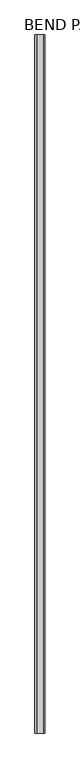
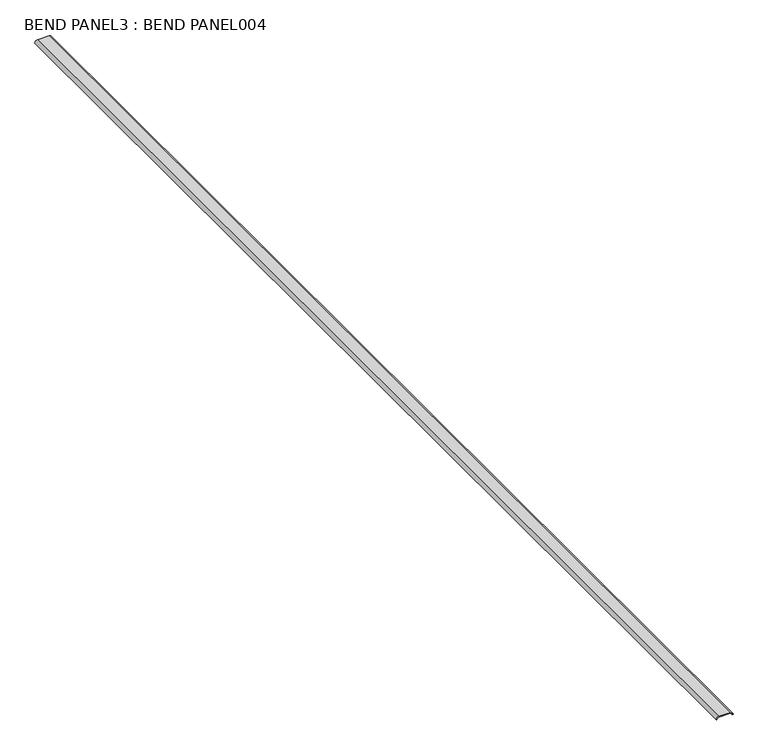
"""IFC4 building model written with IfcOpenShell, lengths in millimetres: proxy geometry, BEND PANEL3 : BEND PANEL004."""

from ifc_helpers import new_model, si_unit, point, frame, frame_2d, origin, place, context, project, spatial, polyline, circle_curve, trimmed, segment, composite_curve, outline, extrude, source, transform, mapped, element, save


def bend_panel3_bend_panel004_15d214a6(model_context):
    return source(origin(), model_context, "Body", "SweptSolid", [
        extrude(outline(composite_curve([segment(polyline([(42576.61192, 5858.4004637), (42576.61192, 5859.5910887)]), True, "CONTINUOUS"), segment(trimmed(circle_curve(frame_2d((42576.6119199, 5862.9993652)), 3.4082764), [point((42576.61192, 5859.5910887))], [point((42580.0201795, 5863.0100787))], True, "CARTESIAN"), True, "CONTINUOUS"), segment(polyline([(42580.0201795, 5863.0100787), (42580.0201963, 5882.3645691)]), True, "CONTINUOUS"), segment(trimmed(circle_curve(frame_2d((42576.6119199, 5882.3645721)), 3.4082764), [point((42580.0201963, 5882.3645691))], [point((42576.61192, 5885.7728485))], True, "CARTESIAN"), True, "CONTINUOUS"), segment(polyline([(42576.61192, 5885.7728485), (42576.61192, 5886.9634735)]), True, "CONTINUOUS"), segment(trimmed(circle_curve(frame_2d((42576.6119199, 5882.3645721)), 4.5989014), [point((42576.61192, 5886.9634735))], [point((42581.2108213, 5882.364568))], False, "CARTESIAN"), True, "CONTINUOUS"), segment(polyline([(42581.2108213, 5882.364568), (42581.2108045, 5863.0118181)]), True, "CONTINUOUS"), segment(trimmed(circle_curve(frame_2d((42576.6119199, 5862.9993652)), 4.5989014), [point((42581.2108045, 5863.0118181))], [point((42576.61192, 5858.4004637))], False, "CARTESIAN"), True, "CONTINUOUS")], self_intersect=False)), frame((0.0, -1052.8906574, 0.0), z_axis=(0.0, 1.0, 0.0), x_axis=(0.0, 0.0, 1.0)), (0.0, 0.0, 1.0), 1999.85),
    ])


if __name__ == "__main__":
    model = new_model("IFC4")
    model_context = context("Model", 3, world=origin())
    ifc_project = project(units=[si_unit("LENGTHUNIT", "METRE", prefix="MILLI")], contexts=[model_context])
    site = spatial("IfcSite", under=ifc_project)
    building = spatial("IfcBuilding", under=site)
    placement = place(None, origin())
    bend_panel3_bend_panel004_shape = bend_panel3_bend_panel004_15d214a6(model_context)
    element("IfcBuildingElementProxy", 1, Name="BEND PANEL3 : BEND PANEL004", ObjectType="BEND PANEL3 : BEND PANEL004", at=placement, inside=building, context=model_context, shape_type="MappedRepresentation", body=[
        mapped(bend_panel3_bend_panel004_shape, transform((0.0, 0.0, 0.0), x_axis=(1.0, 0.0, 0.0), y_axis=(0.0, 1.0, 0.0), z_axis=(0.0, 0.0, 1.0))),
    ])
    save(model, "model.ifc")

# Revit data of these elements
# Type "BEND PANEL3 : BEND PANEL004"
#   NameOverride = "BEND PANEL004"
# Element 1 (IfcBuildingElementProxy, "BEND PANEL3 : BEND PANEL004")
#   Materials on its faces: "METAL PROFILE"
# Materials
#   "METAL PROFILE": class "Unassigned", colour RGB 128 128 128, transparency 0
